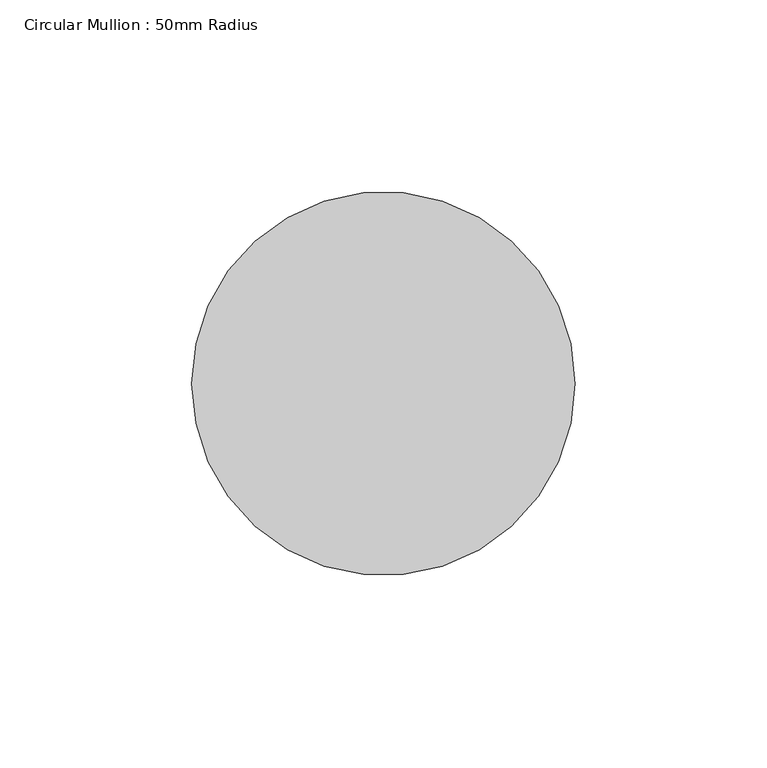
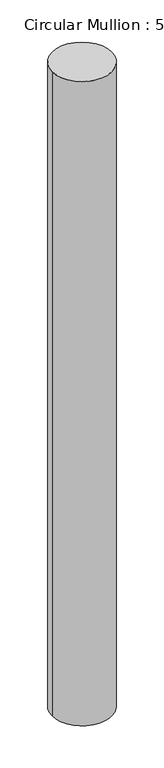
"""IFC4 building model written with IfcOpenShell, lengths in millimetres: member geometry, Circular Mullion : 50mm Radius."""

from ifc_helpers import new_model, si_unit, point, frame, origin, origin_2d, place, context, project, spatial, circle_curve, trimmed, segment, composite_curve, outline, extrude, source, transform, mapped, element, save


def circular_mullion_50mm_radius_3f0050c2(model_context):
    return source(origin(), model_context, "Body", "SweptSolid", [
        extrude(outline(composite_curve([segment(trimmed(circle_curve(origin_2d(), 50.0), [point((50.0, 0.0))], [point((-50.0, 0.0))], False, "CARTESIAN"), True, "CONTINUOUS"), segment(trimmed(circle_curve(origin_2d(), 50.0), [point((-50.0, 0.0))], [point((50.0, 0.0))], False, "CARTESIAN"), True, "CONTINUOUS")], self_intersect=False)), frame((0.0, 0.0, -1142.05975), z_axis=(0.0, 0.0, 1.0), x_axis=(1.0, 0.0, 0.0)), (0.0, 0.0, 1.0), 1142.05975),
    ])


if __name__ == "__main__":
    model = new_model("IFC4")
    model_context = context("Model", 3, world=origin())
    ifc_project = project(units=[si_unit("LENGTHUNIT", "METRE", prefix="MILLI")], contexts=[model_context])
    site = spatial("IfcSite", under=ifc_project)
    building = spatial("IfcBuilding", under=site)
    placement = place(None, origin())
    circular_mullion_50mm_radius_shape = circular_mullion_50mm_radius_3f0050c2(model_context)
    element("IfcMember", 1, ObjectType="Circular Mullion : 50mm Radius", at=placement, inside=building, context=model_context, shape_type="MappedRepresentation", body=[
        mapped(circular_mullion_50mm_radius_shape, transform((0.0, 0.0, 0.0), x_axis=(1.0, 0.0, 0.0), y_axis=(0.0, 1.0, 0.0), z_axis=(0.0, 0.0, 1.0))),
    ])
    save(model, "model.ifc")

# Revit data of these elements
# Type "Circular Mullion : 50mm Radius"
#   built-in parameter 1007350 = 0.164042 (stored number, unit not read)
# Element 1 (IfcMember, "Circular Mullion : 50mm Radius")
#   Materials on its faces: "Aluminium"
# Materials
#   "Aluminium": class "Metal", colour RGB 247 247 247, transparency 0, Description = "Aluminium 6061", Cost = 0
